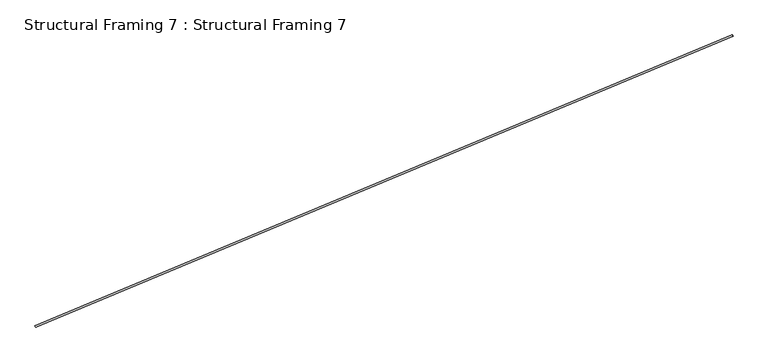
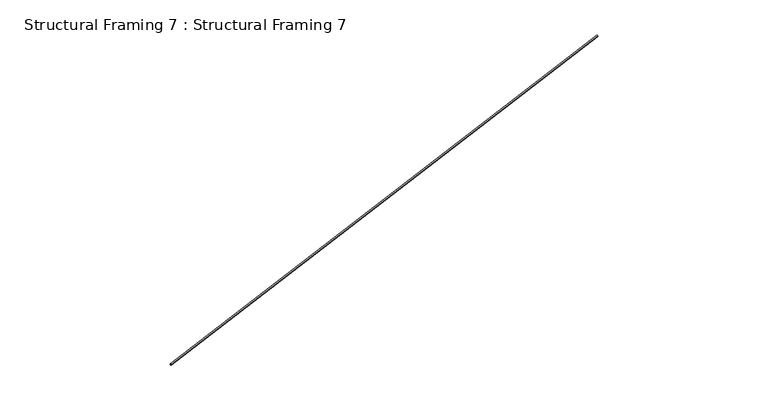
"""IFC4 building model written with IfcOpenShell, lengths in millimetres: beam geometry, Structural Framing 7 : Structural Framing 7."""

from ifc_helpers import new_model, si_unit, point, frame, origin, origin_2d, place, context, project, spatial, circle_curve, trimmed, segment, composite_curve, outline, extrude, source, transform, mapped, element, save


def structural_framing_7_structural_framing_7_1a731511(model_context):
    return source(origin(), model_context, "Body", "SweptSolid", [
        extrude(outline(composite_curve([segment(trimmed(circle_curve(origin_2d(), 6.35), [point((0.0, -6.35))], [point((0.0, 6.3500001))], False, "CARTESIAN"), True, "CONTINUOUS"), segment(trimmed(circle_curve(origin_2d(), 6.35), [point((0.0, 6.3500001))], [point((0.0, -6.35))], False, "CARTESIAN"), True, "CONTINUOUS")], self_intersect=False)), frame((12603.0897681, 282.3662123, 2861.0177297), z_axis=(0.9227531257280362, 0.38510091650472056, 0.014965061522204016), x_axis=(0.0, 0.03883079534680305, -0.9992458002577418)), (0.0, 0.0, 1.0), 5780.5276962),
    ])


if __name__ == "__main__":
    model = new_model("IFC4")
    model_context = context("Model", 3, world=origin())
    ifc_project = project(units=[si_unit("LENGTHUNIT", "METRE", prefix="MILLI")], contexts=[model_context])
    site = spatial("IfcSite", under=ifc_project)
    building = spatial("IfcBuilding", under=site)
    placement = place(None, origin())
    structural_framing_7_structural_framing_7_shape = structural_framing_7_structural_framing_7_1a731511(model_context)
    element("IfcBeam", 1, ObjectType="Structural Framing 7 : Structural Framing 7", at=placement, inside=building, context=model_context, shape_type="MappedRepresentation", body=[
        mapped(structural_framing_7_structural_framing_7_shape, transform((0.0, 0.0, 0.0), x_axis=(1.0, 0.0, 0.0), y_axis=(0.0, 1.0, 0.0), z_axis=(0.0, 0.0, 1.0))),
    ])
    save(model, "model.ifc")

# Revit data of these elements
# Type "Structural Framing 7 : Structural Framing 7"
#   Structural Material [instance default] = EXISTING LATERAL BRACING (1/4" CABLE)
# Element 1 (IfcBeam, "Structural Framing 7 : Structural Framing 7")
#   Materials on its faces: "EXISTING LATERAL BRACING (1/4\" CABLE)"
# Materials
#   "EXISTING LATERAL BRACING (1/4\" CABLE)": class "Generic", colour RGB 120 120 120, transparency 0, Cost = 0
